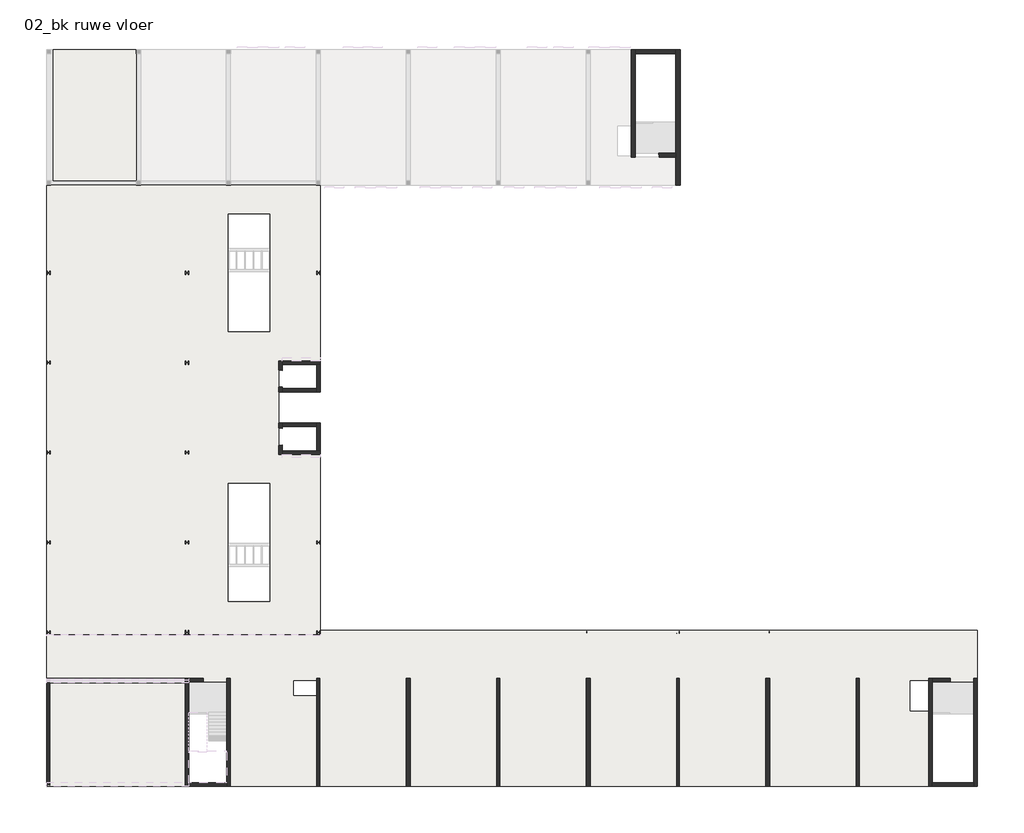
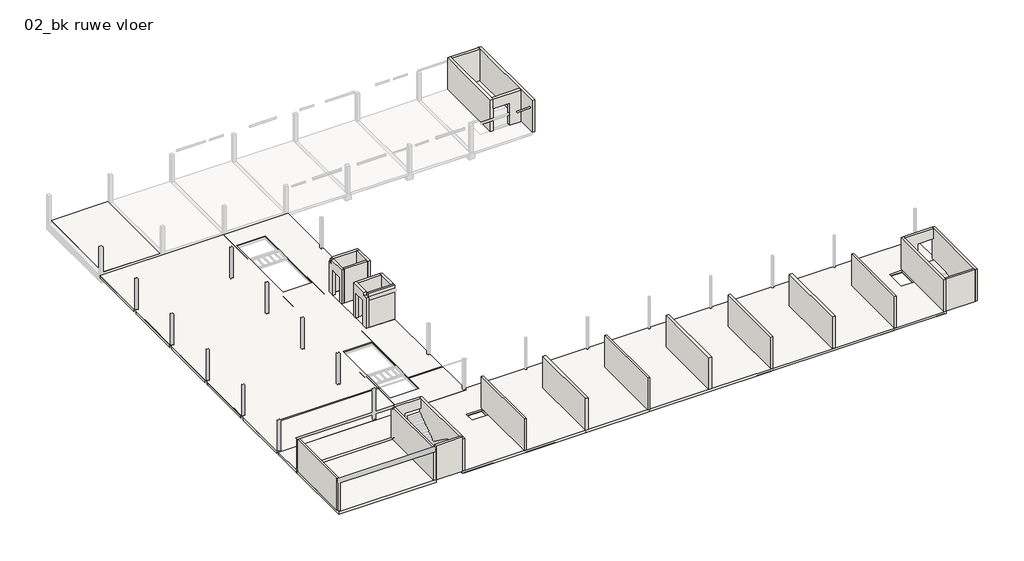
# One storey, part 1 of 3: 28 walls, 20 slabs.
# Revit data of these elements (continued)
# Type "NLRS_22_WA_beton prefab 300_gen_rsf" (continued)
#   IfcExportAs = "IfcWall"
#   Layers, outside or top first: 300 mm "NLRS_f2_beton prefab_gen_rsf" (function 1)
# Type "NLRS_21_WA_beton prefab 300_gen_rsf"
#   Keynote = ""
#   Type IfcGUID = "2ajLwCSRTE_9I1Spg4sCru"
#   Description = "buitenwand beton prefab, generiek"
#   Assembly Code = "21.21"
#   IfcExportAs = "IfcWall"
#   Layers, outside or top first: 300 mm "NLRS_f2_beton prefab_gen_rsf" (function 1)
# Type "NLRS_22_WA_beton prefab 250_gen_rsf"
#   Keynote = ""
#   Type IfcGUID = "2GRbcre991teoKeCLB8LsU"
#   Description = "binnenwand beton prefab, generiek"
#   Assembly Code = "22.21"
#   IfcExportAs = "IfcWall"
#   Layers, outside or top first: 250 mm "NLRS_f2_beton prefab_gen_rsf" (function 1)
# Type "NLRS_21_WA_beton prefab 250_gen_rsf"
#   Keynote = ""
#   Type IfcGUID = "3N5NK1g7D9AwpiDnyE93lX"
#   Description = "buitenwand beton prefab, generiek"
#   Assembly Code = "21.21"
#   IfcExportAs = "IfcWall"
#   Layers, outside or top first: 250 mm "NLRS_f2_beton prefab_gen_rsf" (function 1)
# Element 1 (IfcSlab, "NLRS_23_FL_breedplaat 260_gen_rsf")
#   IfcGUID = "13lTCcCQ95UOWcvnmPh7sO"
#   Comments = ""
#   Height Offset From Level = 0 mm
#   built-in parameter 1001954 = 1
#   IsExternal = no
#   LoadBearing = yes
#   Phase Created = NLRS_nieuw
#   Materials on its faces: "NLRS_f2_beton ihwg_gen_rsf"
# Element 2 (IfcSlab, "NLRS_23_FL_breedplaat 260_gen_rsf")
#   IfcGUID = "13lTCcCQ95UOWcvnmPh7tf"
#   Height Offset From Level = 0 mm
#   built-in parameter 1001954 = 1
#   IsExternal = no
#   LoadBearing = yes
#   Phase Created = NLRS_nieuw
#   Materials on its faces: "NLRS_f2_beton ihwg_gen_rsf"
# Element 3 (IfcSlab, "NLRS_23_FL_druklaag 70_gen_rsf")
#   IfcGUID = "13lTCcCQ95UOWcvnmPh7u_"
#   Height Offset From Level = 0 mm
#   built-in parameter 1001954 = 1
#   IsExternal = no
#   LoadBearing = yes
#   Phase Created = NLRS_nieuw
#   Materials on its faces: "NLRS_f2_beton ihwg_gen_rsf"
# Element 4 (IfcSlab, "NLRS_23_FL_kanaalplaat 260_gen_rsf")
#   IfcGUID = "13lTCcCQ95UOWcvnmPh7v0"
#   built-in parameter 1001955 = -1.5708 (stored number, unit not read)
#   Height Offset From Level = -70 mm
#   built-in parameter 1001954 = 1
#   IsExternal = no
#   LoadBearing = yes
#   Phase Created = NLRS_nieuw
#   Materials on its faces: "NLRS_f2_beton prefab_gen_rsf"
# Element 5 (IfcSlab, "NLRS_23_FL_kanaalplaat 260_gen_rsf")
#   IfcGUID = "13lTCcCQ95UOWcvnmPh7vt"
#   built-in parameter 1001955 = -1.5708 (stored number, unit not read)
#   Height Offset From Level = -70 mm
#   built-in parameter 1001954 = 1
#   IsExternal = no
#   LoadBearing = yes
#   Phase Created = NLRS_nieuw
#   Materials on its faces: "NLRS_f2_beton prefab_gen_rsf"
# Element 6 (IfcSlab, "NLRS_23_FL_kanaalplaat 260_gen_rsf")
#   IfcGUID = "13lTCcCQ95UOWcvnmPh7va"
#   built-in parameter 1001955 = -1.5708 (stored number, unit not read)
#   Height Offset From Level = -70 mm
#   built-in parameter 1001954 = 1
#   IsExternal = no
#   LoadBearing = yes
#   Phase Created = NLRS_nieuw
#   Materials on its faces: "NLRS_f2_beton prefab_gen_rsf"
# Element 7 (IfcSlab, "NLRS_23_FL_kanaalplaat 260_gen_rsf")
#   IfcGUID = "13lTCcCQ95UOWcvnmPh7w3"
#   built-in parameter 1001955 = -1.5708 (stored number, unit not read)
#   Height Offset From Level = -70 mm
#   built-in parameter 1001954 = 1
#   IsExternal = no
#   LoadBearing = yes
#   Phase Created = NLRS_nieuw
#   Materials on its faces: "NLRS_f2_beton prefab_gen_rsf"
# Element 8 (IfcSlab, "NLRS_23_FL_kanaalplaat 260_gen_rsf")
#   IfcGUID = "13lTCcCQ95UOWcvnmPh7ws"
#   built-in parameter 1001955 = 1.5708 (stored number, unit not read)
#   Height Offset From Level = -70 mm
#   built-in parameter 1001954 = 1
#   IsExternal = no
#   LoadBearing = yes
#   Phase Created = NLRS_nieuw
#   Materials on its faces: "NLRS_f2_beton prefab_gen_rsf"
# Element 9 (IfcSlab, "NLRS_23_FL_kanaalplaat 260_gen_rsf")
#   IfcGUID = "13lTCcCQ95UOWcvnmPh7wl"
#   Height Offset From Level = -70 mm
#   built-in parameter 1001954 = 1
#   IsExternal = no
#   LoadBearing = yes
#   Phase Created = NLRS_nieuw
#   Materials on its faces: "NLRS_f2_beton prefab_gen_rsf"
# Element 10 (IfcSlab, "NLRS_23_FL_kanaalplaat 260_gen_rsf")
#   IfcGUID = "13lTCcCQ95UOWcvnmPh7xU"
#   built-in parameter 1001955 = -1.5708 (stored number, unit not read)
#   Height Offset From Level = -70 mm
#   built-in parameter 1001954 = 1
#   IsExternal = no
#   LoadBearing = yes
#   Phase Created = NLRS_nieuw
#   Materials on its faces: "NLRS_f2_beton prefab_gen_rsf"
# Element 11 (IfcSlab, "NLRS_23_FL_kanaalplaat 260_gen_rsf")
#   IfcGUID = "13lTCcCQ95UOWcvnmPh7xJ"
#   built-in parameter 1001955 = 1.5708 (stored number, unit not read)
#   Height Offset From Level = -70 mm
#   built-in parameter 1001954 = 1
#   IsExternal = no
#   LoadBearing = yes
#   Phase Created = NLRS_nieuw
#   Materials on its faces: "NLRS_f2_beton prefab_gen_rsf"
# Element 12 (IfcSlab, "NLRS_23_FL_kanaalplaat 260_gen_rsf")
#   IfcGUID = "13lTCcCQ95UOWcvnmPh7x4"
#   built-in parameter 1001955 = 1.5708 (stored number, unit not read)
#   Height Offset From Level = -70 mm
#   built-in parameter 1001954 = 1
#   IsExternal = no
#   LoadBearing = yes
#   Phase Created = NLRS_nieuw
#   Materials on its faces: "NLRS_f2_beton prefab_gen_rsf"
# Element 13 (IfcSlab, "NLRS_23_FL_kanaalplaat 260_gen_rsf")
#   IfcGUID = "13lTCcCQ95UOWcvnmPh7x$"
#   built-in parameter 1001955 = 1.5708 (stored number, unit not read)
#   Height Offset From Level = -70 mm
#   built-in parameter 1001954 = 1
#   IsExternal = no
#   LoadBearing = yes
#   Phase Created = NLRS_nieuw
#   Materials on its faces: "NLRS_f2_beton prefab_gen_rsf"
# Element 14 (IfcSlab, "NLRS_23_FL_kanaalplaat 260_gen_rsf")
#   IfcGUID = "13lTCcCQ95UOWcvnmPh7xm"
#   built-in parameter 1001955 = -1.5708 (stored number, unit not read)
#   Height Offset From Level = -70 mm
#   built-in parameter 1001954 = 1
#   IsExternal = no
#   LoadBearing = yes
#   Phase Created = NLRS_nieuw
#   Materials on its faces: "NLRS_f2_beton prefab_gen_rsf"
# Element 15 (IfcSlab, "NLRS_23_FL_kanaalplaat 260_gen_rsf")
#   IfcGUID = "13lTCcCQ95UOWcvnmPh7xf"
#   Height Offset From Level = -70 mm
#   built-in parameter 1001954 = 1
#   IsExternal = no
#   LoadBearing = yes
#   Phase Created = NLRS_nieuw
#   Materials on its faces: "NLRS_f2_beton prefab_gen_rsf"
# Element 16 (IfcSlab, "NLRS_23_FL_kanaalplaat 260_gen_rsf")
#   IfcGUID = "13lTCcCQ95UOWcvnmPh7yS"
#   built-in parameter 1001955 = 1.5708 (stored number, unit not read)
#   Height Offset From Level = -70 mm
#   built-in parameter 1001954 = 1
#   IsExternal = no
#   LoadBearing = yes
#   Phase Created = NLRS_nieuw
#   Materials on its faces: "NLRS_f2_beton prefab_gen_rsf"
# Element 17 (IfcSlab, "NLRS_23_FL_breedplaat 260_gen_rsf")
#   IfcGUID = "3aMdMHoe12P9KDGPyaIhfl"
#   built-in parameter 1001955 = 1.5708 (stored number, unit not read)
#   Height Offset From Level = 0 mm
#   built-in parameter 1001954 = 1
#   IsExternal = no
#   LoadBearing = yes
#   Phase Created = NLRS_nieuw
#   Materials on its faces: "NLRS_f2_beton ihwg_gen_rsf"
# Element 18 (IfcSlab, "NLRS_23_FL_breedplaat schil 60_gen_rsf")
#   IfcGUID = "30fJl_yZvFzewSfsmFGxtY"
#   Comments = ""
#   Height Offset From Level = -200 mm
#   built-in parameter 1001954 = 1
#   IsExternal = no
#   LoadBearing = yes
#   Phase Created = NLRS_nieuw
#   Materials on its faces: "NLRS_f2_beton prefab_gen_rsf"
# Element 19 (IfcSlab, "NLRS_23_FL_breedplaat schil 60_gen_rsf")
#   IfcGUID = "2NjBJrSTnArAq_EA_3B3B5"
#   Comments = ""
#   built-in parameter 1001955 = -1.5708 (stored number, unit not read)
#   Height Offset From Level = -200 mm
#   built-in parameter 1001954 = 1
#   IsExternal = no
#   LoadBearing = yes
#   Phase Created = NLRS_nieuw
#   Materials on its faces: "NLRS_f2_beton prefab_gen_rsf"
# Element 20 (IfcSlab, "NLRS_23_FL_breedplaat schil 60_gen_rsf")
#   IfcGUID = "2qE$kEBNbDT8O3EB3ypEdt"
#   Comments = ""
#   Height Offset From Level = -200 mm
#   built-in parameter 1001954 = 1
#   IsExternal = no
#   LoadBearing = yes
#   Phase Created = NLRS_nieuw
#   Materials on its faces: "NLRS_f2_beton prefab_gen_rsf"
# Element 21 (IfcWall, "NLRS_22_WA_beton ihw 250_gen_rsf")
#   IfcGUID = "13lTCcCQ95UOWcvnmPh77b"
#   Comments = ""
#   Top Offset = 0 mm
#   Base Offset = 0 mm
#   wall height = 3540 mm
#   IsExternal = no
#   LoadBearing = yes
#   Phase Created = NLRS_nieuw
#   Base Constraint = 02_bk ruwe vloer
#   Top Constraint = 03_ok ruwe vloer
#   Materials on its faces: "NLRS_f2_beton ihwg_gen_rsf"
# Element 22 (IfcWall, "NLRS_22_WA_beton ihw 250_gen_rsf")
#   IfcGUID = "13lTCcCQ95UOWcvnmPh77d"
#   Comments = ""
#   Top Offset = 0 mm
#   Base Offset = 0 mm
#   wall height = 3540 mm
#   IsExternal = no
#   LoadBearing = yes
#   Phase Created = NLRS_nieuw
#   Base Constraint = 02_bk ruwe vloer
#   Top Constraint = 03_ok ruwe vloer
#   Materials on its faces: "NLRS_f2_beton ihwg_gen_rsf"
# Element 23 (IfcWall, "NLRS_22_WA_kalkzandsteen CS12 214_gen_rsf")
#   IfcGUID = "13lTCcCQ95UOWcvnmPh77X"
#   Comments = ""
#   Top Offset = 0 mm
#   Base Offset = 0 mm
#   wall height = 3540 mm
#   IsExternal = no
#   LoadBearing = yes
#   Phase Created = NLRS_nieuw
#   Base Constraint = 02_bk ruwe vloer
#   Top Constraint = 03_ok ruwe vloer
#   Materials on its faces: "NLRS_f1_kalkzandsteen_gen_rsf"
# Element 24 (IfcWall, "NLRS_22_WA_beton ihw 300_gen_rsf")
#   IfcGUID = "13lTCcCQ95UOWcvnmPh77Z"
#   Comments = ""
#   Top Offset = 0 mm
#   Base Offset = 0 mm
#   wall height = 3540 mm
#   IsExternal = no
#   LoadBearing = yes
#   Phase Created = NLRS_nieuw
#   Base Constraint = 02_bk ruwe vloer
#   Top Constraint = 03_ok ruwe vloer
#   Materials on its faces: "NLRS_f2_beton ihwg_gen_rsf"
# Element 25 (IfcWall, "NLRS_22_WA_kalkzandsteen CS12 214_gen_rsf")
#   IfcGUID = "13lTCcCQ95UOWcvnmPh78T"
#   Comments = ""
#   Top Offset = 0 mm
#   Base Offset = 0 mm
#   wall height = 3540 mm
#   IsExternal = no
#   LoadBearing = yes
#   Phase Created = NLRS_nieuw
#   Base Constraint = 02_bk ruwe vloer
#   Top Constraint = 03_ok ruwe vloer
#   Materials on its faces: "NLRS_f1_kalkzandsteen_gen_rsf"
# Element 26 (IfcWall, "NLRS_22_WA_beton ihw 300_gen_rsf")
#   IfcGUID = "13lTCcCQ95UOWcvnmPh78V"
#   Comments = ""
#   Top Offset = 0 mm
#   Base Offset = 0 mm
#   wall height = 3540 mm
#   IsExternal = no
#   LoadBearing = yes
#   Phase Created = NLRS_nieuw
#   Base Constraint = 02_bk ruwe vloer
#   Top Constraint = 03_ok ruwe vloer
#   Materials on its faces: "NLRS_f2_beton ihwg_gen_rsf"
# Element 27 (IfcWall, "NLRS_22_WA_kalkzandsteen CS12 214_gen_rsf")
#   IfcGUID = "13lTCcCQ95UOWcvnmPh78P"
#   Comments = ""
#   Top Offset = 0 mm
#   Base Offset = 0 mm
#   wall height = 3540 mm
#   IsExternal = no
#   LoadBearing = yes
#   Phase Created = NLRS_nieuw
#   Base Constraint = 02_bk ruwe vloer
#   Top Constraint = 03_ok ruwe vloer
#   Materials on its faces: "NLRS_f1_kalkzandsteen_gen_rsf"
# Element 28 (IfcWall, "NLRS_22_WA_beton ihw 300_gen_rsf")
#   IfcGUID = "13lTCcCQ95UOWcvnmPh78R"
#   Comments = ""
#   Top Offset = 0 mm
#   Base Offset = 0 mm
#   wall height = 3540 mm
#   IsExternal = no
#   LoadBearing = yes
#   Phase Created = NLRS_nieuw
#   Base Constraint = 02_bk ruwe vloer
#   Top Constraint = 03_ok ruwe vloer
#   Materials on its faces: "NLRS_f2_beton ihwg_gen_rsf"
# Element 29 (IfcWall, "NLRS_22_WA_kalkzandsteen CS12 214_gen_rsf")
#   IfcGUID = "13lTCcCQ95UOWcvnmPh78L"
#   Comments = ""
#   Top Offset = 0 mm
#   Base Offset = 0 mm
#   wall height = 3540 mm
#   IsExternal = no
#   LoadBearing = yes
#   Phase Created = NLRS_nieuw
#   Base Constraint = 02_bk ruwe vloer
#   Top Constraint = 03_ok ruwe vloer
#   Materials on its faces: "NLRS_f1_kalkzandsteen_gen_rsf"
# Element 30 (IfcWall, "NLRS_21_WA_beton ihw 250_gen_rsf")
#   IfcGUID = "13lTCcCQ95UOWcvnmPh78N"
#   Comments = ""
#   Top Offset = 0 mm
#   Base Offset = 0 mm
#   wall height = 3540 mm
#   IsExternal = yes
#   LoadBearing = yes
#   Phase Created = NLRS_nieuw
#   Base Constraint = 02_bk ruwe vloer
#   Top Constraint = 03_ok ruwe vloer
#   Materials on its faces: "NLRS_f2_beton ihwg_gen_rsf"
# Element 31 (IfcWall, "NLRS_21_WA_kalkzandsteen CS12 214_gen_rsf")
#   IfcGUID = "13lTCcCQ95UOWcvnmPh78H"
#   Comments = ""
#   Top Offset = 0 mm
#   Base Offset = 0 mm
#   wall height = 3540 mm
#   IsExternal = yes
#   LoadBearing = yes
#   Phase Created = NLRS_nieuw
#   Base Constraint = 02_bk ruwe vloer
#   Top Constraint = 03_ok ruwe vloer
#   Materials on its faces: "NLRS_f1_kalkzandsteen_gen_rsf"
# Element 32 (IfcWall, "NLRS_21_WA_beton ihw 250_gen_rsf")
#   IfcGUID = "13lTCcCQ95UOWcvnmPh78J"
#   Top Offset = 0 mm
#   Base Offset = 0 mm
#   wall height = 3800 mm
#   IsExternal = yes
#   LoadBearing = yes
#   Phase Created = NLRS_nieuw
#   Base Constraint = 02_bk ruwe vloer
#   Top Constraint = 03_bk. ruwe vloer
#   Materials on its faces: "NLRS_f2_beton ihwg_gen_rsf"
# Element 33 (IfcWall, "NLRS_22_WA_beton ihw 250_gen_rsf")
#   IfcGUID = "13lTCcCQ95UOWcvnmPh78D"
#   Top Offset = 0 mm
#   Base Offset = 0 mm
#   wall height = 3540 mm
#   IsExternal = no
#   LoadBearing = yes
#   Phase Created = NLRS_nieuw
#   Base Constraint = 02_bk ruwe vloer
#   Top Constraint = 03_ok ruwe vloer
#   Materials on its faces: "NLRS_f2_beton ihwg_gen_rsf"
# Element 34 (IfcWall, "NLRS_22_WA_beton ihw 250_gen_rsf")
#   IfcGUID = "13lTCcCQ95UOWcvnmPh78F"
#   Comments = ""
#   Top Offset = 0 mm
#   Base Offset = 0 mm
#   wall height = 3540 mm
#   IsExternal = no
#   LoadBearing = yes
#   Phase Created = NLRS_nieuw
#   Base Constraint = 02_bk ruwe vloer
#   Top Constraint = 03_ok ruwe vloer
#   Materials on its faces: "NLRS_f2_beton ihwg_gen_rsf"
# Element 35 (IfcWall, "NLRS_21_WA_beton ihw 250_gen_rsf")
#   IfcGUID = "13lTCcCQ95UOWcvnmPh789"
#   Top Offset = 0 mm
#   Base Offset = 0 mm
#   wall height = 3540 mm
#   IsExternal = yes
#   LoadBearing = yes
#   Phase Created = NLRS_nieuw
#   Base Constraint = 02_bk ruwe vloer
#   Top Constraint = 03_ok ruwe vloer
#   Materials on its faces: "NLRS_f2_beton ihwg_gen_rsf"
# Element 36 (IfcWall, "NLRS_22_WA_beton ihw 250_gen_rsf")
#   IfcGUID = "13lTCcCQ95UOWcvnmPh78B"
#   Top Offset = 0 mm
#   Base Offset = 0 mm
#   wall height = 3540 mm
#   IsExternal = no
#   LoadBearing = yes
#   Phase Created = NLRS_nieuw
#   Base Constraint = 02_bk ruwe vloer
#   Top Constraint = 03_ok ruwe vloer
#   Materials on its faces: "NLRS_f2_beton ihwg_gen_rsf"
# Element 37 (IfcWall, "NLRS_22_WA_beton prefab 300_gen_rsf")
#   IfcGUID = "13lTCcCQ95UOWcvnmPh79n"
#   Comments = ""
#   built-in parameter 1001111 = 20 mm
#   Top Offset = 0 mm
#   Base Offset = 20 mm
#   wall height = 3520 mm
#   IsExternal = no
#   LoadBearing = yes
#   Phase Created = NLRS_nieuw
#   Base Constraint = 02_bk ruwe vloer
#   Top Constraint = 03_ok ruwe vloer
#   Materials on its faces: "NLRS_f2_beton prefab_gen_rsf"
# Element 38 (IfcWall, "NLRS_21_WA_beton prefab 300_gen_rsf")
#   IfcGUID = "13lTCcCQ95UOWcvnmPh79k"
#   Comments = ""
#   built-in parameter 1001111 = 20 mm
#   Top Offset = 0 mm
#   Base Offset = 20 mm
#   wall height = 3520 mm
#   IsExternal = yes
#   LoadBearing = yes
#   Phase Created = NLRS_nieuw
#   Base Constraint = 02_bk ruwe vloer
#   Top Constraint = 03_ok ruwe vloer
#   Materials on its faces: "NLRS_f2_beton prefab_gen_rsf"
# Element 39 (IfcWall, "NLRS_21_WA_beton prefab 300_gen_rsf")
#   IfcGUID = "13lTCcCQ95UOWcvnmPh79e"
#   Comments = ""
#   built-in parameter 1001111 = 20 mm
#   Top Offset = 0 mm
#   Base Offset = 20 mm
#   wall height = 3520 mm
#   IsExternal = yes
#   LoadBearing = yes
#   Phase Created = NLRS_nieuw
#   Base Constraint = 02_bk ruwe vloer
#   Top Constraint = 03_ok ruwe vloer
#   Materials on its faces: "NLRS_f2_beton prefab_gen_rsf"
# Element 40 (IfcWall, "NLRS_22_WA_beton prefab 300_gen_rsf")
#   IfcGUID = "13lTCcCQ95UOWcvnmPh79g"
#   Comments = ""
#   built-in parameter 1001111 = 20 mm
#   Top Offset = 0 mm
#   Base Offset = 20 mm
#   wall height = 3520 mm
#   IsExternal = no
#   LoadBearing = yes
#   Phase Created = NLRS_nieuw
#   Base Constraint = 02_bk ruwe vloer
#   Top Constraint = 03_ok ruwe vloer
#   Materials on its faces: "NLRS_f2_beton prefab_gen_rsf"
# Element 41 (IfcWall, "NLRS_22_WA_beton prefab 250_gen_rsf")
#   IfcGUID = "13lTCcCQ95UOWcvnmPh7B5"
#   built-in parameter 1001111 = 20 mm
#   Top Offset = 0 mm
#   Base Offset = 20 mm
#   wall height = 3780 mm
#   IsExternal = no
#   LoadBearing = yes
#   Phase Created = NLRS_nieuw
#   Base Constraint = 02_bk ruwe vloer
#   Top Constraint = 03_bk. ruwe vloer
#   Materials on its faces: "NLRS_f2_beton prefab_gen_rsf"
# Element 42 (IfcWall, "NLRS_22_WA_beton prefab 250_gen_rsf")
#   IfcGUID = "13lTCcCQ95UOWcvnmPh7B7"
#   built-in parameter 1001111 = 20 mm
#   Top Offset = 0 mm
#   Base Offset = 20 mm
#   wall height = 3780 mm
#   IsExternal = no
#   LoadBearing = yes
#   Phase Created = NLRS_nieuw
#   Base Constraint = 02_bk ruwe vloer
#   Top Constraint = 03_bk. ruwe vloer
#   Materials on its faces: "NLRS_f2_beton prefab_gen_rsf"
# Element 43 (IfcWall, "NLRS_22_WA_beton prefab 250_gen_rsf")
#   IfcGUID = "13lTCcCQ95UOWcvnmPh7B1"
#   built-in parameter 1001111 = 20 mm
#   Top Offset = 0 mm
#   Base Offset = 20 mm
#   wall height = 3780 mm
#   IsExternal = no
#   LoadBearing = yes
#   Phase Created = NLRS_nieuw
#   Base Constraint = 02_bk ruwe vloer
#   Top Constraint = 03_bk. ruwe vloer
#   Materials on its faces: "NLRS_f2_beton prefab_gen_rsf"
# Element 44 (IfcWall, "NLRS_21_WA_beton prefab 250_gen_rsf")
#   IfcGUID = "13lTCcCQ95UOWcvnmPh7B3"
#   built-in parameter 1001111 = 20 mm
#   Top Offset = 0 mm
#   Base Offset = 20 mm
#   wall height = 3780 mm
#   IsExternal = yes
#   LoadBearing = yes
#   Phase Created = NLRS_nieuw
#   Base Constraint = 02_bk ruwe vloer
#   Top Constraint = 03_bk. ruwe vloer
#   Materials on its faces: "NLRS_f2_beton prefab_gen_rsf"
# Element 45 (IfcWall, "NLRS_22_WA_beton prefab 250_gen_rsf")
#   IfcGUID = "13lTCcCQ95UOWcvnmPh7Bz"
#   built-in parameter 1001111 = 20 mm
#   Top Offset = 0 mm
#   Base Offset = 20 mm
#   wall height = 3780 mm
#   IsExternal = no
#   LoadBearing = yes
#   Phase Created = NLRS_nieuw
#   Base Constraint = 02_bk ruwe vloer
#   Top Constraint = 03_bk. ruwe vloer
#   Materials on its faces: "NLRS_f2_beton prefab_gen_rsf"
# Element 46 (IfcWall, "NLRS_22_WA_beton prefab 250_gen_rsf")
#   IfcGUID = "13lTCcCQ95UOWcvnmPh7B$"
#   built-in parameter 1001111 = 20 mm
#   Top Offset = 0 mm
#   Base Offset = 20 mm
#   wall height = 3780 mm
#   IsExternal = no
#   LoadBearing = yes
#   Phase Created = NLRS_nieuw
#   Base Constraint = 02_bk ruwe vloer
#   Top Constraint = 03_bk. ruwe vloer
#   Materials on its faces: "NLRS_f2_beton prefab_gen_rsf"
# Element 47 (IfcWall, "NLRS_22_WA_beton prefab 250_gen_rsf")
#   IfcGUID = "13lTCcCQ95UOWcvnmPh7Bv"
#   built-in parameter 1001111 = 20 mm
#   Top Offset = 0 mm
#   Base Offset = 20 mm
#   wall height = 3780 mm
#   IsExternal = no
#   LoadBearing = yes
#   Phase Created = NLRS_nieuw
#   Base Constraint = 02_bk ruwe vloer
#   Top Constraint = 03_bk. ruwe vloer
#   Materials on its faces: "NLRS_f2_beton prefab_gen_rsf"
# Element 48 (IfcWall, "NLRS_21_WA_beton prefab 250_gen_rsf")
#   IfcGUID = "13lTCcCQ95UOWcvnmPh7Bx"
#   built-in parameter 1001111 = 20 mm
#   Top Offset = 0 mm
#   Base Offset = 20 mm
#   wall height = 3780 mm
#   IsExternal = yes
#   LoadBearing = yes
#   Phase Created = NLRS_nieuw
#   Base Constraint = 02_bk ruwe vloer
#   Top Constraint = 03_bk. ruwe vloer
#   Materials on its faces: "NLRS_f2_beton prefab_gen_rsf"
# Materials
#   "NLRS_f2_beton ihwg_gen_rsf": class "F - Niet gebakken kunststeen", colour RGB 129 133 118, transparency 0, Keynote = "f2", Manufacturer = "Revit Standards Foundation", URL = "www.revitstandards.org", Description = "beton ihwg", Cost = 0
#   "NLRS_f2_beton prefab_gen_rsf": class "F - Niet gebakken kunststeen", colour RGB 129 133 118, transparency 0, Keynote = "f2", Manufacturer = "Revit Standards Foundation", URL = "www.revitstandards.org", Description = "beton prefab", Cost = 0
#   "NLRS_f1_kalkzandsteen_gen_rsf": class "F - Niet gebakken kunststeen", colour RGB 223 221 219, transparency 0, Keynote = "f1", Manufacturer = "Revit Standards Foundation", URL = "www.revitstandards.org", Description = "kalkzandsteen", Cost = 0
